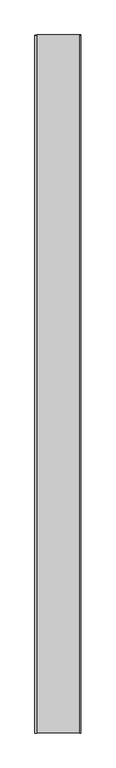
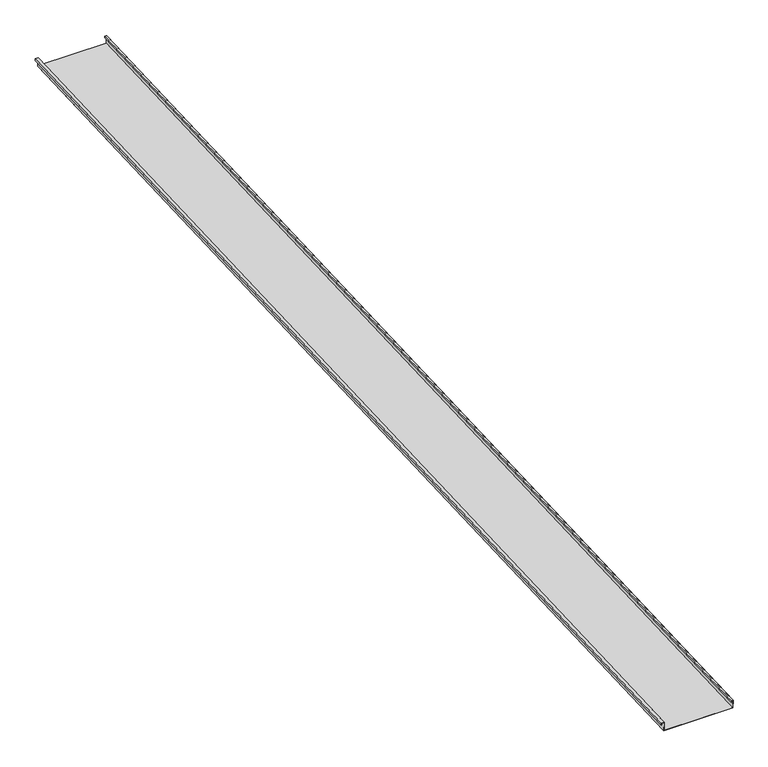
"""IFC4 building model written with IfcOpenShell, lengths in millimetres: proxy geometry, Generic Models 2:Generic Models 2:310765:Generic Models 2:310765 : Generic Models 2:Generic Models 2:310765:97 : Generic Models 2:Generic Models 2:310765:Generic Models 2:310765 : Generic Models 2:Generic Models 2:310765:300385."""

from ifc_helpers import new_model, si_unit, frame, origin, place, context, project, spatial, polyline, outline, extrude, source, transform, mapped, element, save


def generic_models_7ff7a445(model_context):
    return source(origin(), model_context, "Body", "SweptSolid", [
        extrude(outline(polyline([(1.5875, 0.0), (1.5875, 50.8), (407.9875, 50.8), (407.9875, 1.5875), (396.875, 1.5875), (396.875, 11.1125), (398.4625, 11.1125), (398.4625, 3.175), (406.4, 3.175), (406.4, 49.2125), (3.175, 49.2125), (3.175, -1.5874999), (-14.2875, -1.5874999), (-14.2875, 9.525), (-12.7, 9.525), (-12.7, 0.0), (1.5875, 0.0)])), frame((613553.5263073, -581354.4345603, 3902.6697972), z_axis=(0.0, 0.9991330730923568, 0.041630544712067834), x_axis=(1.0, 0.0, 0.0)), (0.0, 0.0, 1.0), 6400.8),
    ])


if __name__ == "__main__":
    model = new_model("IFC4")
    model_context = context("Model", 3, world=origin())
    ifc_project = project(units=[si_unit("LENGTHUNIT", "METRE", prefix="MILLI")], contexts=[model_context])
    site = spatial("IfcSite", under=ifc_project)
    building = spatial("IfcBuilding", under=site)
    placement = place(None, origin())
    generic_models_shape = generic_models_7ff7a445(model_context)
    element("IfcBuildingElementProxy", 1, Name="Generic Models 2:Generic Models 2:310765:Generic Models 2:310765 : Generic Models 2:Generic Models 2:310765:97 : Generic Models 2:Generic Models 2:310765:Generic Models 2:310765 : Generic Models 2:Generic Models 2:310765:300385", ObjectType="Generic Models 2:Generic Models 2:310765:Generic Models 2:310765 : Generic Models 2:Generic Models 2:310765:97 : Generic Models 2:Generic Models 2:310765:Generic Models 2:310765 : Generic Models 2:Generic Models 2:310765:300385", at=placement, inside=building, context=model_context, shape_type="MappedRepresentation", body=[
        mapped(generic_models_shape, transform((0.0, 0.0, 0.0), x_axis=(1.0, 0.0, 0.0), y_axis=(0.0, 1.0, 0.0), z_axis=(0.0, 0.0, 1.0))),
    ])
    save(model, "model.ifc")

# Revit data of these elements
# Type "Generic Models 2:Generic Models 2:310765:Generic Models 2:310765 : Generic Models 2:Generic Models 2:310765:97 : Generic Models 2:Generic Models 2:310765:Generic Models 2:310765 : Generic Models 2:Generic Models 2:310765:300385"
#   NameOverride = "Generic Models 2:Generic Models 2:310765:Generic Models 2:310765 : Generic Models 2:Generic Models 2:310765:300385"
#   ObjectTypeOverride = "Generic Models 2:310765 : Generic Models 2:Generic Models 2:310765"
#   Reference = "Generic Models 2"
#   Tag = "300385"
# Element 1 (IfcBuildingElementProxy, "Generic Models 2:Generic Models 2:310765:Generic Models 2:310765 : Generic Models 2:Generic Models 2:310765:97 : Generic Models 2:Generic Models 2:310765:Generic Models 2:310765 : Generic Models 2:Generic Models 2:310765:300385")
#   Materials on its faces: "THERMAL BROKEN ALUMINUM STOREFRONT FOR POLYCARBONATE"
# Materials
#   "THERMAL BROKEN ALUMINUM STOREFRONT FOR POLYCARBONATE": class "Unassigned", colour RGB 244 244 244, transparency 0, Keynote = "M07611300.01", Cost = 0
